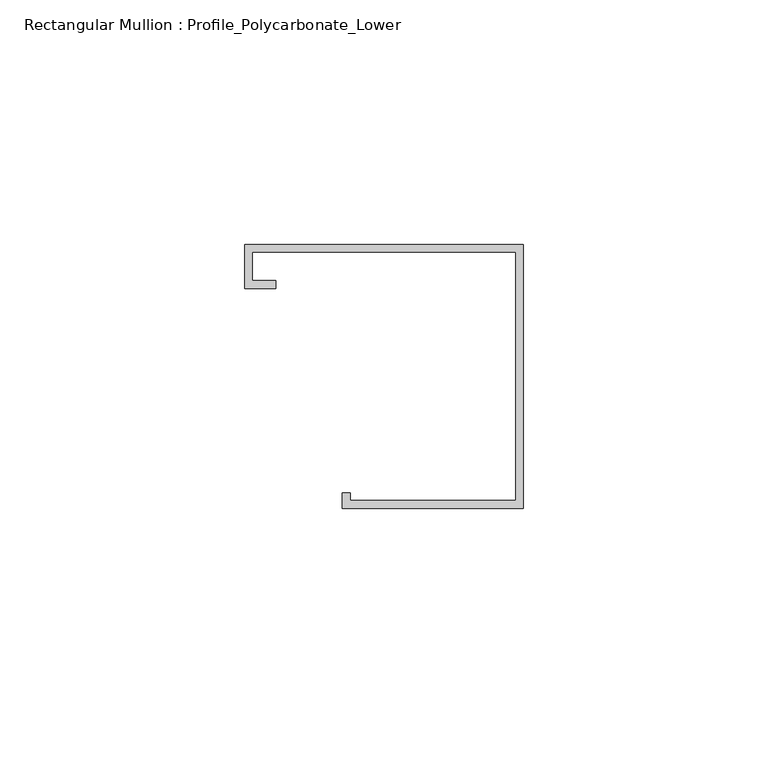
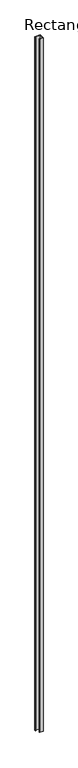
"""IFC4 building model written with IfcOpenShell, lengths in millimetres: member geometry, Rectangular Mullion : Profile_Polycarbonate_Lower."""

from ifc_helpers import new_model, si_unit, frame, origin, place, context, project, spatial, polyline, outline, extrude, source, transform, mapped, element, save


def rectangular_mullion_profile_polycarbonate_lower_a6ffc67b(model_context):
    return source(origin(), model_context, "Body", "SweptSolid", [
        extrude(outline(polyline([(0.0, 28.984575), (0.0, -25.015825), (-36.9824, -25.015825), (-36.9824, -21.840825), (-35.3949, -21.840825), (-35.3949, -23.428325), (-1.5875, -23.428325), (-1.5875, 27.397075), (-55.4101, 27.397075), (-55.4101, 21.580475), (-50.6476, 21.580475), (-50.6476, 19.992975), (-56.9976, 19.992975), (-56.9976, 28.984575), (0.0, 28.984575)])), frame((0.0, 0.0, -7918.6024), z_axis=(0.0, 0.0, 1.0), x_axis=(1.0, 0.0, 0.0)), (0.0, 0.0, 1.0), 7918.6024),
    ])


if __name__ == "__main__":
    model = new_model("IFC4")
    model_context = context("Model", 3, world=origin())
    ifc_project = project(units=[si_unit("LENGTHUNIT", "METRE", prefix="MILLI")], contexts=[model_context])
    site = spatial("IfcSite", under=ifc_project)
    building = spatial("IfcBuilding", under=site)
    placement = place(None, origin())
    rectangular_mullion_profile_polycarbonate_lower_shape = rectangular_mullion_profile_polycarbonate_lower_a6ffc67b(model_context)
    element("IfcMember", 1, ObjectType="Rectangular Mullion : Profile_Polycarbonate_Lower", at=placement, inside=building, context=model_context, shape_type="MappedRepresentation", body=[
        mapped(rectangular_mullion_profile_polycarbonate_lower_shape, transform((0.0, 0.0, 0.0), x_axis=(1.0, 0.0, 0.0), y_axis=(0.0, 1.0, 0.0), z_axis=(0.0, 0.0, 1.0))),
    ])
    save(model, "model.ifc")

# Revit data of these elements
# Type "Rectangular Mullion : Profile_Polycarbonate_Lower"
#   built-in parameter 1007322 = 0.177167 (stored number, unit not read)
#   built-in parameter 1007321 = 0 (stored number, unit not read)
#   built-in parameter 1007320 = 0.00520833 (stored number, unit not read)
